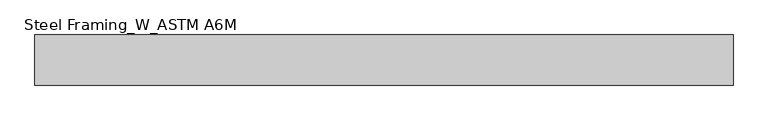
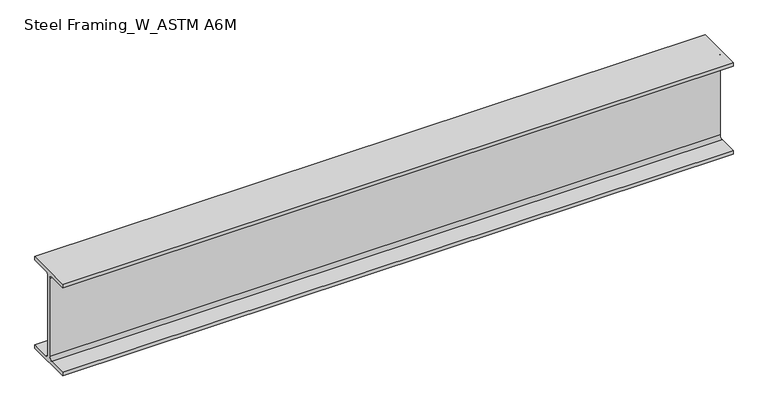
"""IFC4 building model written with IfcOpenShell, lengths in millimetres: beam geometry, Steel Framing_W_ASTM A6M : H_SB_AR_S02_W200x22.5_B7."""

import ifcopenshell
import ifcopenshell.guid

model = None  # the IFC model being written
_history = None  # IfcOwnerHistory: only IFC2X3 demands one
_inside = {}  # id of a spatial element -> (the spatial element, [elements in it])
_under = {}  # id of a project, library or spatial element -> (it, [spatial elements below it])
_declared = {}  # id of a project -> (the project, [libraries it declares])
_typed = {}  # id of a type object -> (the type object, [elements of that type])
_made_of = {}  # id of a material, layer set ... -> (it, [elements and type objects made of it])


def new_model(schema):
    """Start an empty IFC model of exactly this schema.

    Asked for "IFC4X3", IfcOpenShell would pick the latest addendum, in which some entities
    have other attributes; the version numbers below select the first issue.
    IFC2X3 requires an IfcOwnerHistory on every rooted entity: one is made here for all.
    """
    global model, _history
    if schema == "IFC4X3":
        model = ifcopenshell.file(schema_version=(4, 3, 0, 0))
    else:
        model = ifcopenshell.file(schema=schema)
    _inside.clear()
    _under.clear()
    _declared.clear()
    _typed.clear()
    _made_of.clear()
    _history = None
    if model.schema == "IFC2X3":
        org = make("IfcOrganization", Name="unknown")
        user = make(
            "IfcPersonAndOrganization",
            ThePerson=make("IfcPerson", FamilyName="unknown"),
            TheOrganization=org,
        )
        app = make(
            "IfcApplication",
            ApplicationDeveloper=org,
            Version="unknown",
            ApplicationFullName="unknown",
            ApplicationIdentifier="unknown",
        )
        _history = make(
            "IfcOwnerHistory",
            OwningUser=user,
            OwningApplication=app,
            ChangeAction="ADDED",
            CreationDate=0,
        )
    return model


def make(cls, **values):
    """One entity of the class cls with the attributes given. An attribute that is None is left unset."""
    return model.create_entity(
        cls, **{name: value for name, value in values.items() if value is not None}
    )


def rooted(cls, **values):
    """An entity with a GlobalId (a new one), such as an element, a storey or a relation."""
    return make(cls, GlobalId=ifcopenshell.guid.new(), OwnerHistory=_history, **values)


def si_unit(unit_type, name, prefix=None):
    """IfcSIUnit, for example si_unit("LENGTHUNIT", "METRE", prefix="MILLI")."""
    return make("IfcSIUnit", UnitType=unit_type, Prefix=prefix, Name=name)


def assignment(units):
    """IfcUnitAssignment: the units of a project."""
    return None if units is None else make("IfcUnitAssignment", Units=units)


def point(xyz):
    """IfcCartesianPoint."""
    return None if xyz is None else make("IfcCartesianPoint", Coordinates=xyz)


def direction(xyz):
    """IfcDirection."""
    return None if xyz is None else make("IfcDirection", DirectionRatios=xyz)


def frame(location, z_axis=None, x_axis=None):
    """IfcAxis2Placement3D, a coordinate frame: its origin and axes. An axis left out is left unset."""
    return make(
        "IfcAxis2Placement3D",
        Location=point(location),
        Axis=direction(z_axis),
        RefDirection=direction(x_axis),
    )


def frame_2d(location, x_axis=None):
    """IfcAxis2Placement2D, a coordinate frame in the plane: its origin and x axis."""
    return make(
        "IfcAxis2Placement2D", Location=point(location), RefDirection=direction(x_axis)
    )


def origin():
    """The frame at (0, 0, 0) with its axes left unset."""
    return frame((0.0, 0.0, 0.0))


def place(relative_to, where):
    """IfcLocalPlacement: puts the frame where relative to a parent placement (None: the world)."""
    return make(
        "IfcLocalPlacement", PlacementRelTo=relative_to, RelativePlacement=where
    )


def context(
    kind, dimensions, precision=None, world=None, true_north=None, identifier=None
):
    """IfcGeometricRepresentationContext, for example the 3D "Model" context."""
    return make(
        "IfcGeometricRepresentationContext",
        ContextIdentifier=identifier,
        ContextType=kind,
        CoordinateSpaceDimension=dimensions,
        Precision=precision,
        WorldCoordinateSystem=world,
        TrueNorth=true_north,
    )


def project(units=None, contexts=None):
    """IfcProject with its units and contexts."""
    return rooted(
        "IfcProject",
        Name="project",
        RepresentationContexts=contexts,
        UnitsInContext=assignment(units),
    )


def spatial(cls, under=None, at=None, **own):
    """A site, building, storey or space (cls), placed at a placement, below another one or the project."""
    s = rooted(cls, ObjectPlacement=at, **own)
    if under is not None:
        _under.setdefault(under.id(), (under, []))[1].append(s)
    return s


def polyline(points):
    """IfcPolyline through the points."""
    return make("IfcPolyline", Points=[point(p) for p in points])


def circle_curve(where, radius):
    """IfcCircle in the frame where."""
    return make("IfcCircle", Position=where, Radius=radius)


def trimmed(basis, trim1, trim2, sense, master):
    """IfcTrimmedCurve: the piece of a basis curve between two trims."""
    return make(
        "IfcTrimmedCurve",
        BasisCurve=basis,
        Trim1=trim1,
        Trim2=trim2,
        SenseAgreement=sense,
        MasterRepresentation=master,
    )


def segment(curve, same_sense, transition):
    """IfcCompositeCurveSegment."""
    return make(
        "IfcCompositeCurveSegment",
        Transition=transition,
        SameSense=same_sense,
        ParentCurve=curve,
    )


def composite_curve(segments, self_intersect=None):
    """IfcCompositeCurve: segments joined end to end."""
    return make("IfcCompositeCurve", Segments=segments, SelfIntersect=self_intersect)


def outline(outer, holes=None, kind="AREA"):
    """IfcArbitraryClosedProfileDef: a profile drawn as a closed curve; with holes, ...WithVoids."""
    if holes is None:
        return make("IfcArbitraryClosedProfileDef", ProfileType=kind, OuterCurve=outer)
    return make(
        "IfcArbitraryProfileDefWithVoids",
        ProfileType=kind,
        OuterCurve=outer,
        InnerCurves=holes,
    )


def extrude(swept, where, along, depth):
    """IfcExtrudedAreaSolid: the profile swept, set in the frame where, extruded along a direction by depth."""
    return make(
        "IfcExtrudedAreaSolid",
        SweptArea=swept,
        Position=where,
        ExtrudedDirection=direction(along),
        Depth=depth,
    )


def shape(context_of_items, identifier, shape_type, items):
    """IfcShapeRepresentation: the items that make up one representation, for example the "Body"."""
    return make(
        "IfcShapeRepresentation",
        ContextOfItems=context_of_items,
        RepresentationIdentifier=identifier,
        RepresentationType=shape_type,
        Items=items,
    )


def source(mapping_origin, context_of_items, identifier, shape_type, items):
    """IfcRepresentationMap: a shape defined once, which mapped items show again and again."""
    return make(
        "IfcRepresentationMap",
        MappingOrigin=mapping_origin,
        MappedRepresentation=shape(context_of_items, identifier, shape_type, items),
    )


def transform(
    local_origin,
    x_axis=None,
    y_axis=None,
    z_axis=None,
    scale=None,
    scale2=None,
    scale3=None,
    uniform=True,
):
    """IfcCartesianTransformationOperator3D, or its non-uniform kind. x_axis, y_axis, z_axis: its Axis1, 2, 3."""
    if uniform:
        return make(
            "IfcCartesianTransformationOperator3D",
            Axis1=direction(x_axis),
            Axis2=direction(y_axis),
            LocalOrigin=point(local_origin),
            Scale=scale,
            Axis3=direction(z_axis),
        )
    return make(
        "IfcCartesianTransformationOperator3DnonUniform",
        Axis1=direction(x_axis),
        Axis2=direction(y_axis),
        LocalOrigin=point(local_origin),
        Scale=scale,
        Axis3=direction(z_axis),
        Scale2=scale2,
        Scale3=scale3,
    )


def mapped(mapping_source, mapping_target):
    """IfcMappedItem: shows the shape of a source again, moved by a transform."""
    return make(
        "IfcMappedItem", MappingSource=mapping_source, MappingTarget=mapping_target
    )


def made_of(thing, what):
    """Note that an element or type object is made of a material, layer set ...; save() writes the relation."""
    if what is not None:
        _made_of.setdefault(what.id(), (what, []))[1].append(thing)
    return thing


def element(
    cls,
    number,
    at=None,
    inside=None,
    cuts=None,
    type_object=None,
    material=None,
    context=None,
    identifier="Body",
    shape_type=None,
    held_by="IfcProductDefinitionShape",
    body=None,
    shapes=None,
    **own,
):
    """One element of the class cls, such as IfcWall. Its Tag is "e" and its number.

    at: its placement. inside: the storey or other place that contains it. cuts: it is an
    opening in that element (IfcRelVoidsElement). A single representation is given by context,
    identifier, shape_type and body (its items); several are given by shapes. held_by: the class
    of the entity that holds the representations. save() writes the other relations.
    """
    e = rooted(cls, Tag="e%d" % number, ObjectPlacement=at, **own)
    if body is not None:
        shapes = [shape(context, identifier, shape_type, body)]
    if shapes is not None:
        e.Representation = make(held_by, Representations=shapes)
    if inside is not None:
        _inside.setdefault(inside.id(), (inside, []))[1].append(e)
    if cuts is not None:
        rooted(
            "IfcRelVoidsElement", RelatingBuildingElement=cuts, RelatedOpeningElement=e
        )
    if type_object is not None:
        _typed.setdefault(type_object.id(), (type_object, []))[1].append(e)
    return made_of(e, material)


def aggregate(whole, parts):
    """IfcRelAggregates: a whole, such as a stair, and the parts it consists of."""
    return rooted("IfcRelAggregates", RelatingObject=whole, RelatedObjects=parts)


def save(model, path):
    """Write the relations noted so far, then the file.

    IfcRelAggregates (storeys below a building ...), IfcRelContainedInSpatialStructure (elements
    in a storey), IfcRelDefinesByType, IfcRelAssociatesMaterial and IfcRelDeclares: one each for
    every whole, place, type object, material and project.
    """
    for whole, parts in _under.values():
        aggregate(whole, parts)
    for where, things in _inside.values():
        rooted(
            "IfcRelContainedInSpatialStructure",
            RelatedElements=things,
            RelatingStructure=where,
        )
    for kind, things in _typed.values():
        rooted("IfcRelDefinesByType", RelatedObjects=things, RelatingType=kind)
    for what, things in _made_of.values():
        rooted("IfcRelAssociatesMaterial", RelatedObjects=things, RelatingMaterial=what)
    for by, libraries in _declared.values():
        rooted("IfcRelDeclares", RelatingContext=by, RelatedDefinitions=libraries)
    model.write(path)


def steel_framing_w_astm_a6m_b276909d(model_context):
    return source(origin(), model_context, "Body", "SweptSolid", [
        extrude(outline(composite_curve([segment(polyline([(51.0, -95.0), (51.0, -103.0), (-51.0, -103.0), (-51.0, -95.0), (-10.71, -95.0)]), True, "CONTINUOUS"), segment(trimmed(circle_curve(frame_2d((-10.71, -87.4)), 7.6), [point((-10.71, -95.0))], [point((-3.11, -87.4))], True, "CARTESIAN"), True, "CONTINUOUS"), segment(polyline([(-3.11, -87.4), (-3.11, 87.4)]), True, "CONTINUOUS"), segment(trimmed(circle_curve(frame_2d((-10.71, 87.4)), 7.6), [point((-3.11, 87.4))], [point((-10.71, 95.0))], True, "CARTESIAN"), True, "CONTINUOUS"), segment(polyline([(-10.71, 95.0), (-51.0, 95.0), (-51.0, 103.0), (51.0, 103.0), (51.0, 95.0), (10.71, 95.0)]), True, "CONTINUOUS"), segment(trimmed(circle_curve(frame_2d((10.71, 87.4)), 7.6), [point((10.71, 95.0))], [point((3.11, 87.4))], True, "CARTESIAN"), True, "CONTINUOUS"), segment(polyline([(3.11, 87.4), (3.11, -87.4)]), True, "CONTINUOUS"), segment(trimmed(circle_curve(frame_2d((10.71, -87.4)), 7.6), [point((3.11, -87.4))], [point((10.71, -95.0))], True, "CARTESIAN"), True, "CONTINUOUS"), segment(polyline([(10.71, -95.0), (51.0, -95.0)]), True, "CONTINUOUS")], self_intersect=False)), frame((-710.3, 0.0, 0.0), z_axis=(1.0, 0.0, 0.0), x_axis=(0.0, 1.0, 0.0)), (0.0, 0.0, 1.0), 1420.6),
    ])


if __name__ == "__main__":
    model = new_model("IFC4")
    model_context = context("Model", 3, world=origin())
    ifc_project = project(units=[si_unit("LENGTHUNIT", "METRE", prefix="MILLI")], contexts=[model_context])
    site = spatial("IfcSite", under=ifc_project)
    building = spatial("IfcBuilding", under=site)
    placement = place(None, origin())
    steel_framing_w_astm_a6m_shape = steel_framing_w_astm_a6m_b276909d(model_context)
    element("IfcBeam", 1, ObjectType="Steel Framing_W_ASTM A6M : H_SB_AR_S02_W200x22.5_B7", at=placement, inside=building, context=model_context, shape_type="MappedRepresentation", body=[
        mapped(steel_framing_w_astm_a6m_shape, transform((0.0, 0.0, 0.0), x_axis=(1.0, 0.0, 0.0), y_axis=(0.0, 1.0, 0.0), z_axis=(0.0, 0.0, 1.0))),
    ])
    save(model, "model.ifc")

# Revit data of these elements
# Type "Steel Framing_W_ASTM A6M : H_SB_AR_S02_W200x22.5_B7"
#   Section Name Key = "W8x15"
#   Width = 10.2 cm
#   Web Thickness = 0.622 cm
#   Web Fillet = 0.76 cm
#   Warping Constant = 13900.0 cm⁶
#   Torsional Moment of Inertia = 5.70 cm⁴
#   Section Area = 28.6 cm²
#   Plastic Modulus weak axis = 43.8 cm³
#   Plastic Modulus strong axis = 223.0 cm³
#   Perimeter = 0.795 m²/m
#   Nominal Weight = 22.50 kgf/m
#   Moment of Inertia weak axis = 142.00 cm⁴
#   Moment of Inertia strong axis = 2000.00 cm⁴
#   Height = 20.6 cm
#   Flange Thickness = 0.8 cm
#   Elastic Modulus weak axis = 27.9 cm³
#   Elastic Modulus strong axis = 193.0 cm³
#   Centroid Vertical = 10.3 cm
#   Centroid Horizontal = 5.1 cm
#   Length [instance default] = 1500 mm
#   Structural Material [instance default] = Steel, 45-345
#   Bolt Spacing = 0
#   Assembly Code = ""
# Element 1 (IfcBeam, "Steel Framing_W_ASTM A6M : H_SB_AR_S02_W200x22.5_B7")
#   Materials on its faces: "Steel, 45-345"
# Materials
#   "Steel, 45-345": class "Metal", colour RGB 189 187 185, transparency 0, Description = "Steel 345 MPa", Cost = 0
